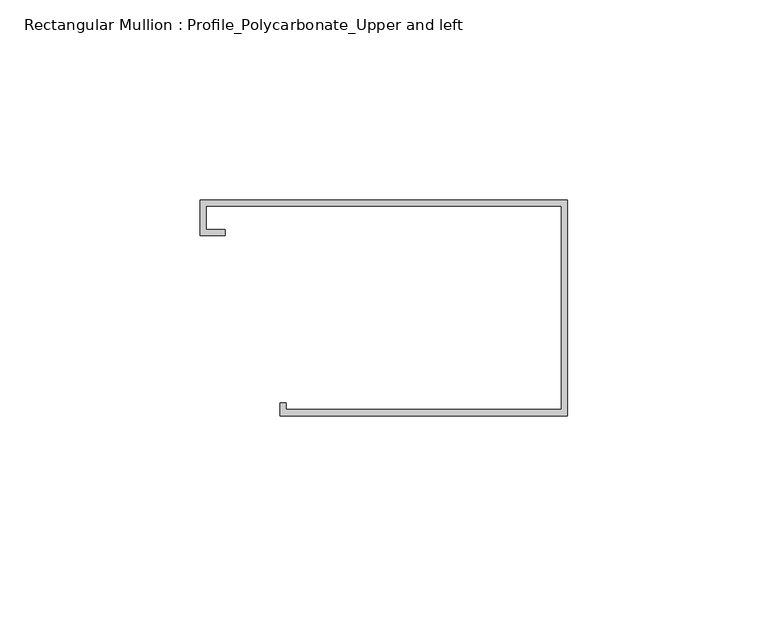
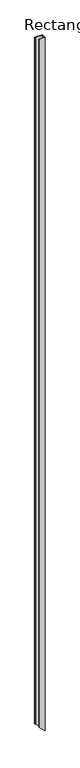
"""IFC4 building model written with IfcOpenShell, lengths in millimetres: member geometry, Rectangular Mullion : Profile_Polycarbonate_Upper and left."""

import ifcopenshell
import ifcopenshell.guid

model = None  # the IFC model being written
_history = None  # IfcOwnerHistory: only IFC2X3 demands one
_inside = {}  # id of a spatial element -> (the spatial element, [elements in it])
_under = {}  # id of a project, library or spatial element -> (it, [spatial elements below it])
_declared = {}  # id of a project -> (the project, [libraries it declares])
_typed = {}  # id of a type object -> (the type object, [elements of that type])
_made_of = {}  # id of a material, layer set ... -> (it, [elements and type objects made of it])


def new_model(schema):
    """Start an empty IFC model of exactly this schema.

    Asked for "IFC4X3", IfcOpenShell would pick the latest addendum, in which some entities
    have other attributes; the version numbers below select the first issue.
    IFC2X3 requires an IfcOwnerHistory on every rooted entity: one is made here for all.
    """
    global model, _history
    if schema == "IFC4X3":
        model = ifcopenshell.file(schema_version=(4, 3, 0, 0))
    else:
        model = ifcopenshell.file(schema=schema)
    _inside.clear()
    _under.clear()
    _declared.clear()
    _typed.clear()
    _made_of.clear()
    _history = None
    if model.schema == "IFC2X3":
        org = make("IfcOrganization", Name="unknown")
        user = make(
            "IfcPersonAndOrganization",
            ThePerson=make("IfcPerson", FamilyName="unknown"),
            TheOrganization=org,
        )
        app = make(
            "IfcApplication",
            ApplicationDeveloper=org,
            Version="unknown",
            ApplicationFullName="unknown",
            ApplicationIdentifier="unknown",
        )
        _history = make(
            "IfcOwnerHistory",
            OwningUser=user,
            OwningApplication=app,
            ChangeAction="ADDED",
            CreationDate=0,
        )
    return model


def make(cls, **values):
    """One entity of the class cls with the attributes given. An attribute that is None is left unset."""
    return model.create_entity(
        cls, **{name: value for name, value in values.items() if value is not None}
    )


def rooted(cls, **values):
    """An entity with a GlobalId (a new one), such as an element, a storey or a relation."""
    return make(cls, GlobalId=ifcopenshell.guid.new(), OwnerHistory=_history, **values)


def si_unit(unit_type, name, prefix=None):
    """IfcSIUnit, for example si_unit("LENGTHUNIT", "METRE", prefix="MILLI")."""
    return make("IfcSIUnit", UnitType=unit_type, Prefix=prefix, Name=name)


def assignment(units):
    """IfcUnitAssignment: the units of a project."""
    return None if units is None else make("IfcUnitAssignment", Units=units)


def point(xyz):
    """IfcCartesianPoint."""
    return None if xyz is None else make("IfcCartesianPoint", Coordinates=xyz)


def direction(xyz):
    """IfcDirection."""
    return None if xyz is None else make("IfcDirection", DirectionRatios=xyz)


def frame(location, z_axis=None, x_axis=None):
    """IfcAxis2Placement3D, a coordinate frame: its origin and axes. An axis left out is left unset."""
    return make(
        "IfcAxis2Placement3D",
        Location=point(location),
        Axis=direction(z_axis),
        RefDirection=direction(x_axis),
    )


def origin():
    """The frame at (0, 0, 0) with its axes left unset."""
    return frame((0.0, 0.0, 0.0))


def place(relative_to, where):
    """IfcLocalPlacement: puts the frame where relative to a parent placement (None: the world)."""
    return make(
        "IfcLocalPlacement", PlacementRelTo=relative_to, RelativePlacement=where
    )


def context(
    kind, dimensions, precision=None, world=None, true_north=None, identifier=None
):
    """IfcGeometricRepresentationContext, for example the 3D "Model" context."""
    return make(
        "IfcGeometricRepresentationContext",
        ContextIdentifier=identifier,
        ContextType=kind,
        CoordinateSpaceDimension=dimensions,
        Precision=precision,
        WorldCoordinateSystem=world,
        TrueNorth=true_north,
    )


def project(units=None, contexts=None):
    """IfcProject with its units and contexts."""
    return rooted(
        "IfcProject",
        Name="project",
        RepresentationContexts=contexts,
        UnitsInContext=assignment(units),
    )


def spatial(cls, under=None, at=None, **own):
    """A site, building, storey or space (cls), placed at a placement, below another one or the project."""
    s = rooted(cls, ObjectPlacement=at, **own)
    if under is not None:
        _under.setdefault(under.id(), (under, []))[1].append(s)
    return s


def faces_of(points, faces, orient=None, outer=None):
    """IfcFace entities. A face is a list of loops; a loop is a list of indices into points, from 0.

    orient and outer hold one flag for each loop. By default every Orientation is true, the
    first loop of a face is its IfcFaceOuterBound and the others are IfcFaceBound.
    """
    made = []
    for i, loops in enumerate(faces):
        bounds = []
        for j, loop in enumerate(loops):
            is_outer = j == 0 if outer is None else outer[i][j]
            bounds.append(
                make(
                    "IfcFaceOuterBound" if is_outer else "IfcFaceBound",
                    Bound=make("IfcPolyLoop", Polygon=[points[k] for k in loop]),
                    Orientation=True if orient is None else orient[i][j],
                )
            )
        made.append(make("IfcFace", Bounds=bounds))
    return made


def faceted_brep(points, faces, orient=None, outer=None, voids=None):
    """IfcFacetedBrep: a solid bounded by flat faces; with voids (closed shells), ...WithVoids."""
    shared = [point(p) for p in points]
    hull = make("IfcClosedShell", CfsFaces=faces_of(shared, faces, orient, outer))
    if voids is None:
        return make("IfcFacetedBrep", Outer=hull)
    return make(
        "IfcFacetedBrepWithVoids",
        Outer=hull,
        Voids=[
            make(cls, CfsFaces=faces_of(shared, fs, o, b)) for cls, fs, o, b in voids
        ],
    )


def shape(context_of_items, identifier, shape_type, items):
    """IfcShapeRepresentation: the items that make up one representation, for example the "Body"."""
    return make(
        "IfcShapeRepresentation",
        ContextOfItems=context_of_items,
        RepresentationIdentifier=identifier,
        RepresentationType=shape_type,
        Items=items,
    )


def source(mapping_origin, context_of_items, identifier, shape_type, items):
    """IfcRepresentationMap: a shape defined once, which mapped items show again and again."""
    return make(
        "IfcRepresentationMap",
        MappingOrigin=mapping_origin,
        MappedRepresentation=shape(context_of_items, identifier, shape_type, items),
    )


def transform(
    local_origin,
    x_axis=None,
    y_axis=None,
    z_axis=None,
    scale=None,
    scale2=None,
    scale3=None,
    uniform=True,
):
    """IfcCartesianTransformationOperator3D, or its non-uniform kind. x_axis, y_axis, z_axis: its Axis1, 2, 3."""
    if uniform:
        return make(
            "IfcCartesianTransformationOperator3D",
            Axis1=direction(x_axis),
            Axis2=direction(y_axis),
            LocalOrigin=point(local_origin),
            Scale=scale,
            Axis3=direction(z_axis),
        )
    return make(
        "IfcCartesianTransformationOperator3DnonUniform",
        Axis1=direction(x_axis),
        Axis2=direction(y_axis),
        LocalOrigin=point(local_origin),
        Scale=scale,
        Axis3=direction(z_axis),
        Scale2=scale2,
        Scale3=scale3,
    )


def mapped(mapping_source, mapping_target):
    """IfcMappedItem: shows the shape of a source again, moved by a transform."""
    return make(
        "IfcMappedItem", MappingSource=mapping_source, MappingTarget=mapping_target
    )


def made_of(thing, what):
    """Note that an element or type object is made of a material, layer set ...; save() writes the relation."""
    if what is not None:
        _made_of.setdefault(what.id(), (what, []))[1].append(thing)
    return thing


def element(
    cls,
    number,
    at=None,
    inside=None,
    cuts=None,
    type_object=None,
    material=None,
    context=None,
    identifier="Body",
    shape_type=None,
    held_by="IfcProductDefinitionShape",
    body=None,
    shapes=None,
    **own,
):
    """One element of the class cls, such as IfcWall. Its Tag is "e" and its number.

    at: its placement. inside: the storey or other place that contains it. cuts: it is an
    opening in that element (IfcRelVoidsElement). A single representation is given by context,
    identifier, shape_type and body (its items); several are given by shapes. held_by: the class
    of the entity that holds the representations. save() writes the other relations.
    """
    e = rooted(cls, Tag="e%d" % number, ObjectPlacement=at, **own)
    if body is not None:
        shapes = [shape(context, identifier, shape_type, body)]
    if shapes is not None:
        e.Representation = make(held_by, Representations=shapes)
    if inside is not None:
        _inside.setdefault(inside.id(), (inside, []))[1].append(e)
    if cuts is not None:
        rooted(
            "IfcRelVoidsElement", RelatingBuildingElement=cuts, RelatedOpeningElement=e
        )
    if type_object is not None:
        _typed.setdefault(type_object.id(), (type_object, []))[1].append(e)
    return made_of(e, material)


def aggregate(whole, parts):
    """IfcRelAggregates: a whole, such as a stair, and the parts it consists of."""
    return rooted("IfcRelAggregates", RelatingObject=whole, RelatedObjects=parts)


def save(model, path):
    """Write the relations noted so far, then the file.

    IfcRelAggregates (storeys below a building ...), IfcRelContainedInSpatialStructure (elements
    in a storey), IfcRelDefinesByType, IfcRelAssociatesMaterial and IfcRelDeclares: one each for
    every whole, place, type object, material and project.
    """
    for whole, parts in _under.values():
        aggregate(whole, parts)
    for where, things in _inside.values():
        rooted(
            "IfcRelContainedInSpatialStructure",
            RelatedElements=things,
            RelatingStructure=where,
        )
    for kind, things in _typed.values():
        rooted("IfcRelDefinesByType", RelatedObjects=things, RelatingType=kind)
    for what, things in _made_of.values():
        rooted("IfcRelAssociatesMaterial", RelatedObjects=things, RelatingMaterial=what)
    for by, libraries in _declared.values():
        rooted("IfcRelDeclares", RelatingContext=by, RelatedDefinitions=libraries)
    model.write(path)


def rectangular_mullion_profile_polycarbonate_upper_and_left_32227215(model_context):
    return source(origin(), model_context, "Body", "Brep", [
        faceted_brep([(0.0, 28.984575, 0.0), (-91.9988, 28.984575, 0.0), (-91.9988, 19.992975, 0.0), (-85.6488, 19.992975, 0.0), (-85.6488, 21.580475, 0.0), (-90.4113, 21.580475, 0.0), (-90.4113, 27.397075, 0.0), (-1.5875, 27.397075, 0.0), (-1.5875, -23.428325, 0.0), (-70.3961, -23.428325, 0.0), (-70.3961, -21.840825, 0.0), (-71.9836, -21.840825, 0.0), (-71.9836, -25.015825, 0.0), (0.0, -25.015825, 0.0), (0.0, 28.984575, -8800.3886628), (-91.9988, 28.984575, -8712.1433207), (-91.9988, 19.992975, -8712.1433207), (-85.6488, 19.992975, -8718.2342471), (-85.6488, 21.580475, -8718.2342471), (-90.4113, 21.580475, -8713.6660523), (-90.4113, 27.397075, -8713.6660523), (-1.5875, 27.397075, -8798.8659312), (-1.5875, -23.428325, -8798.8659312), (-70.3961, -23.428325, -8732.8646524), (-70.3961, -21.840825, -8732.8646524), (-71.9836, -21.840825, -8731.3419208), (-71.9836, -25.015825, -8731.3419208), (0.0, -25.015825, -8800.3886628)], [[[0, 1, 2, 3, 4, 5, 6, 7, 8, 9, 10, 11, 12, 13]], [[1, 0, 14, 15]], [[2, 1, 15, 16]], [[3, 2, 16, 17]], [[4, 3, 17, 18]], [[5, 4, 18, 19]], [[6, 5, 19, 20]], [[7, 6, 20, 21]], [[8, 7, 21, 22]], [[9, 8, 22, 23]], [[10, 9, 23, 24]], [[11, 10, 24, 25]], [[12, 11, 25, 26]], [[13, 12, 26, 27]], [[0, 13, 27, 14]], [[14, 27, 26, 25, 24, 23, 22, 21, 20, 19, 18, 17, 16, 15]]]),
    ])


if __name__ == "__main__":
    model = new_model("IFC4")
    model_context = context("Model", 3, world=origin())
    ifc_project = project(units=[si_unit("LENGTHUNIT", "METRE", prefix="MILLI")], contexts=[model_context])
    site = spatial("IfcSite", under=ifc_project)
    building = spatial("IfcBuilding", under=site)
    placement = place(None, origin())
    rectangular_mullion_profile_polycarbonate_upper_and_left_shape = rectangular_mullion_profile_polycarbonate_upper_and_left_32227215(model_context)
    element("IfcMember", 1, ObjectType="Rectangular Mullion : Profile_Polycarbonate_Upper and left", at=placement, inside=building, context=model_context, shape_type="MappedRepresentation", body=[
        mapped(rectangular_mullion_profile_polycarbonate_upper_and_left_shape, transform((0.0, 0.0, 0.0), x_axis=(1.0, 0.0, 0.0), y_axis=(0.0, 1.0, 0.0), z_axis=(0.0, 0.0, 1.0))),
    ])
    save(model, "model.ifc")

# Revit data of these elements
# Type "Rectangular Mullion : Profile_Polycarbonate_Upper and left"
#   built-in parameter 1007322 = 0.177167 (stored number, unit not read)
#   built-in parameter 1007321 = 0.00520833 (stored number, unit not read)
#   built-in parameter 1007320 = 0 (stored number, unit not read)
